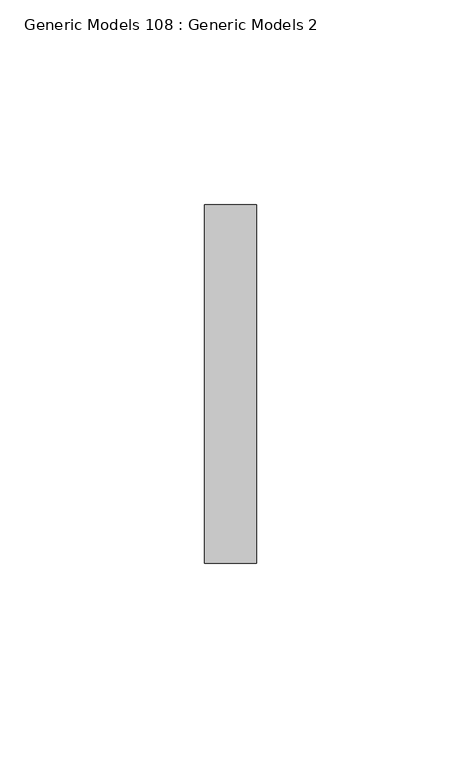
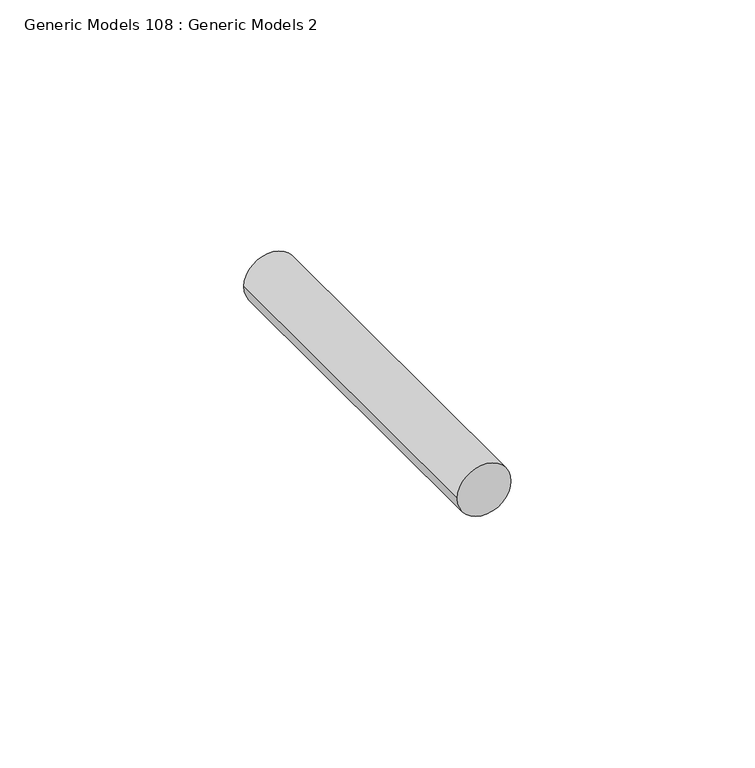
"""IFC4 building model written with IfcOpenShell, lengths in millimetres: proxy geometry, Generic Models 108 : Generic Models 2."""

from ifc_helpers import new_model, si_unit, point, frame, frame_2d, origin, place, context, project, spatial, circle_curve, trimmed, segment, composite_curve, outline, extrude, source, transform, mapped, element, save


def generic_models_108_generic_models_2_bf106c77(model_context):
    return source(origin(), model_context, "Body", "SweptSolid", [
        extrude(outline(composite_curve([segment(trimmed(circle_curve(frame_2d((37517.3905034, 6179.9346014)), 6.35), [point((37517.3905034, 6186.2846014))], [point((37517.3905034, 6173.5846014))], False, "CARTESIAN"), True, "CONTINUOUS"), segment(trimmed(circle_curve(frame_2d((37517.3905034, 6179.9346014)), 6.35), [point((37517.3905034, 6173.5846014))], [point((37517.3905034, 6186.2846014))], False, "CARTESIAN"), True, "CONTINUOUS")], self_intersect=False)), frame((0.0, 1848.3666731, 0.0), z_axis=(0.0, 1.0, 0.0), x_axis=(0.0, 0.0, 1.0)), (0.0, 0.0, 1.0), 87.551022),
    ])


if __name__ == "__main__":
    model = new_model("IFC4")
    model_context = context("Model", 3, world=origin())
    ifc_project = project(units=[si_unit("LENGTHUNIT", "METRE", prefix="MILLI")], contexts=[model_context])
    site = spatial("IfcSite", under=ifc_project)
    building = spatial("IfcBuilding", under=site)
    placement = place(None, origin())
    generic_models_108_generic_models_2_shape = generic_models_108_generic_models_2_bf106c77(model_context)
    element("IfcBuildingElementProxy", 1, Name="Generic Models 108 : Generic Models 2", ObjectType="Generic Models 108 : Generic Models 2", at=placement, inside=building, context=model_context, shape_type="MappedRepresentation", body=[
        mapped(generic_models_108_generic_models_2_shape, transform((0.0, 0.0, 0.0), x_axis=(1.0, 0.0, 0.0), y_axis=(0.0, 1.0, 0.0), z_axis=(0.0, 0.0, 1.0))),
    ])
    save(model, "model.ifc")

# Revit data of these elements
# Element 1 (IfcBuildingElementProxy, "Generic Models 108 : Generic Models 2")
#   Materials on its faces: "S.S. LAG BOLT - SEE STRUCT. DWGS"
# Materials
#   "S.S. LAG BOLT - SEE STRUCT. DWGS": class "Generic", colour RGB 120 120 120, transparency 0, Cost = 0
